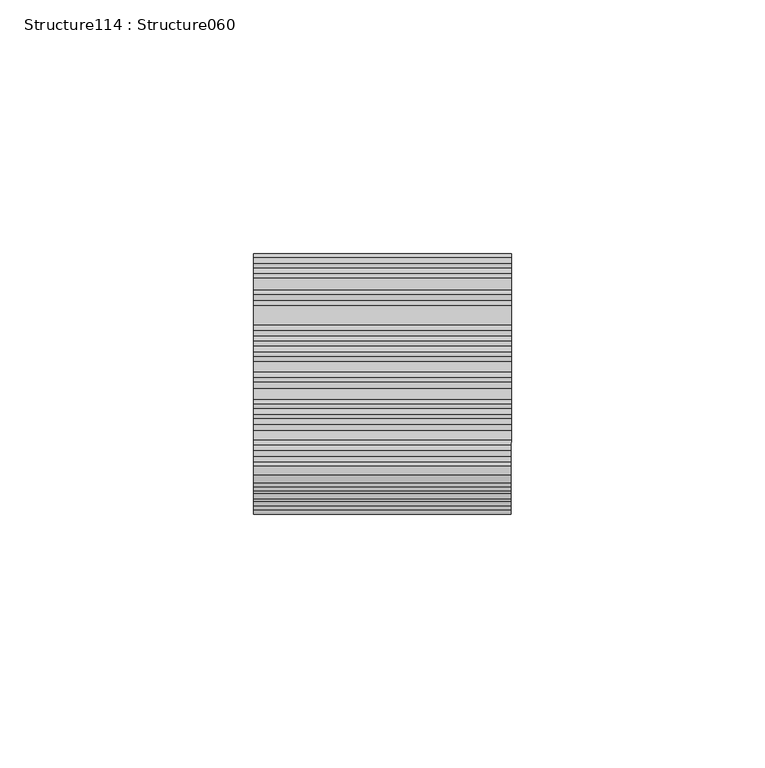
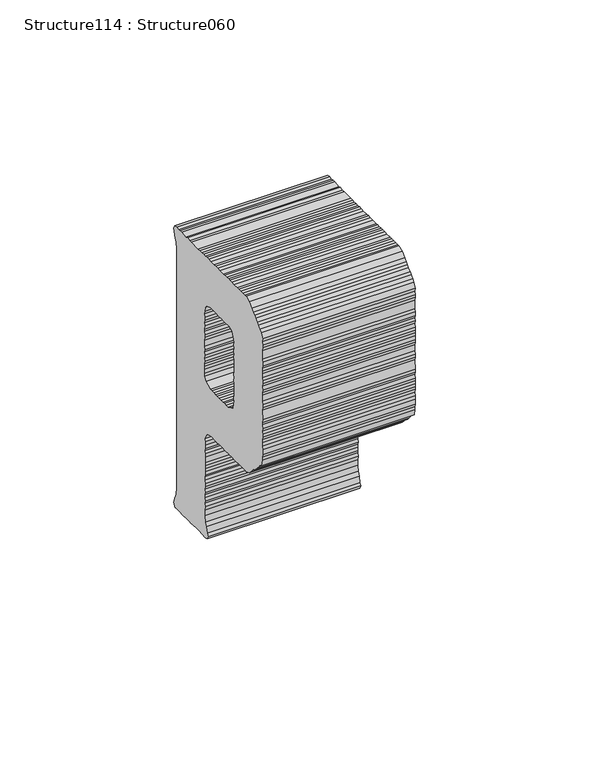
"""IFC4 building model written with IfcOpenShell, lengths in millimetres: proxy geometry, Structure114 : Structure060."""

from ifc_helpers import new_model, si_unit, frame, origin, place, context, project, spatial, polyline, outline, extrude, source, transform, mapped, element, save


def structure114_structure060_e718248d(model_context):
    return source(origin(), model_context, "Body", "SweptSolid", [
        extrude(outline(polyline([(1.9520053, 0.0), (3.1183694, 0.256899), (4.0274787, 0.1273821), (5.3272738, 0.0), (7.4077286, 0.0), (8.3171937, 0.256899), (9.226303, 0.0), (10.3976485, 0.256899), (11.1736827, 0.1273821), (12.3446724, 0.1273821), (13.516018, 0.0), (15.4630419, 0.1273821), (16.3725071, 0.1273821), (17.5434968, 0.256899), (18.7098608, 0.1273821), (19.7477754, 0.1273821), (20.5284353, 0.256899), (22.3470097, -0.5248282), (23.9086852, -1.9537844), (24.6847194, -2.8628937), (25.4703606, -3.5097668), (25.9894958, -4.1623329), (27.0270546, -4.9380113), (27.5461898, -5.7240084), (28.4552992, -6.6270688), (29.2363148, -7.2796349), (30.0119931, -8.9708273), (29.7550941, -10.1368356), (30.0119931, -11.3028439), (30.0119931, -12.0884851), (29.7550941, -13.2541376), (29.7550941, -16.2447692), (30.0119931, -17.2833954), (30.0119931, -18.5824788), (29.7550941, -19.4972812), (29.8835436, -20.4006974), (29.7550941, -21.4396795), (29.8835436, -22.7441001), (30.0119931, -23.6535653), (30.0119931, -24.6864985), (29.8835436, -25.7286829), (30.0119931, -27.0277663), (29.8835436, -28.0667483), (29.7550941, -28.9797716), (29.7550941, -31.0609381), (30.0119931, -32.0931596), (30.0119931, -33.264861), (29.7550941, -34.307757), (30.0119931, -37.425059), (29.8835436, -38.5932022), (29.7550941, -39.3731504), (30.0119931, -40.6722338), (29.8835436, -41.5777849), (30.0119931, -42.6199693), (30.0119931, -43.6585956), (29.8835436, -44.5680607), (29.7550941, -45.7376272), (29.8835436, -46.9096843), (30.0119931, -47.9479548), (30.0119931, -49.7665292), (29.7550941, -50.8090694), (29.7550941, -51.8455608), (29.3647643, -53.9228132), (28.3268497, -54.4458624), (27.8080702, -55.2218966), (26.2463948, -57.0401153), (25.5938287, -57.6926814), (24.5562699, -58.2121724), (23.2564748, -59.7681548), (22.3470097, -60.8103392), (20.5284353, -61.4589914), (19.7477754, -61.3298302), (18.5814114, -61.1963993), (16.3725071, -61.1963993), (15.3345925, -61.4589914), (14.2920522, -61.3298302), (13.2541376, -61.4589914), (12.473122, -61.3298302), (11.1736827, -61.3298302), (10.2642176, -61.1963993), (9.0978535, -61.4589914), (8.3171937, -61.3298302), (7.0173987, -61.1963993), (5.0703747, -61.1963993), (3.8990292, -61.4589914), (2.9899199, -61.3298302), (2.0804548, -61.3298302), (1.0425402, -61.1963993), (-0.2618804, -61.4589914), (-1.9470239, -61.9763475), (-2.4661592, -62.6289136), (-3.246819, -64.320106), (-2.9849385, -65.2292153), (-3.1183694, -66.5243847), (-2.9849385, -67.566925), (-3.246819, -68.4760343), (-2.9849385, -69.3854994), (-3.1183694, -70.6845828), (-3.1183694, -72.6362323), (-2.9849385, -73.6748586), (-3.1183694, -74.7134848), (-3.1183694, -75.7499762), (-2.9849385, -76.9216775), (-3.246819, -77.7016257), (-3.246819, -78.8694131), (-2.9849385, -79.9062602), (-3.1183694, -81.0818755), (-3.246819, -81.9870709), (-2.9849385, -83.1587722), (-3.246819, -83.9387204), (-3.246819, -84.9773466), (-3.1183694, -86.270737), (-3.246819, -87.0563782), (-2.9849385, -88.0950045), (-3.246819, -89.3940879), (-3.246819, -91.3421792), (-2.9849385, -93.4229899), (-2.3377097, -94.7163802), (-1.9470239, -96.7975467), (-1.4282446, -97.579274), (-1.9470239, -98.6157653), (-2.9849385, -98.8783574), (-5.1988244, -98.8783574), (-6.3651884, -98.7491962), (-7.2746536, -98.6157653), (-8.0553134, -98.6157653), (-10.3926672, -98.8783574), (-11.3021323, -98.8783574), (-12.3400469, -98.7491962), (-13.2491562, -98.8783574), (-14.2920522, -98.7491962), (-15.4584164, -98.8783574), (-16.5009566, -98.8783574), (-17.2769908, -98.7491962), (-19.4858951, -98.7491962), (-20.3953603, -98.8783574), (-21.1760201, -97.579274), (-20.9191211, -96.7975467), (-20.5287912, -95.7606995), (-20.009656, -94.4594812), (-19.8762251, -93.6798889), (-19.4858951, -91.3421792), (-19.4858951, -90.4327141), (-19.619326, -89.2667058), (-19.619326, -88.3519035), (-19.3574456, -87.3150563), (-19.619326, -86.1472689), (-19.619326, -85.2342456), (-19.3574456, -84.3286945), (-19.3574456, -83.2865101), (-19.4858951, -81.9870709), (-19.4858951, -81.0818755), (-19.3574456, -80.0393353), (-19.4858951, -79.130226), (-19.619326, -78.0876858), (-19.3574456, -76.7886024), (-19.619326, -75.8830513), (-19.619326, -74.970028), (-19.4858951, -73.9314017), (-19.4858951, -72.6362323), (-19.619326, -71.723209), (-19.4858951, -70.5572007), (-19.3574456, -69.5185745), (-19.4858951, -68.7386263), (-19.4858951, -67.7000001), (-19.3574456, -66.3952236), (-19.3574456, -64.4474881), (-19.4858951, -63.5380229), (-19.619326, -62.3684565), (-19.4858951, -61.1963993), (-19.3574456, -59.1212817), (-19.619326, -58.2121724), (-19.4858951, -57.0401153), (-19.619326, -56.136699), (-19.619326, -54.0558883), (-19.4858951, -53.1407302), (-19.4858951, -51.9747219), (-19.3574456, -50.9364514), (-19.619326, -49.8939112), (-19.3574456, -48.8570641), (-19.619326, -47.9479548), (-19.3574456, -46.6470923), (-19.619326, -45.6102451), (-19.4858951, -44.8285179), (-19.3574456, -43.5294345), (-19.3574456, -41.5777849), (-19.619326, -40.6722338), (-19.4858951, -39.3731504), (-19.3574456, -38.3302544), (-19.3574456, -37.2919839), (-19.4858951, -36.2551368), (-19.4858951, -32.2265905), (-19.3574456, -31.3135673), (-19.619326, -30.1457799), (-19.4858951, -29.2363148), (-19.619326, -27.9372314), (-19.3574456, -26.90074), (-19.4858951, -25.9916307), (-19.3574456, -25.0803865), (-19.3574456, -21.7001367), (-19.4858951, -20.6632895), (-19.4858951, -19.8812064), (-19.3574456, -18.71164), (-19.619326, -17.5438526), (-19.4858951, -16.6343875), (-19.4858951, -14.4258389), (-19.619326, -13.5170855), (-19.619326, -11.4362748), (-19.3574456, -10.5268097), (-19.619326, -9.2334193), (-19.3574456, -7.4091519), (-19.8762251, -5.0714422), (-20.266555, -4.032816), (-20.5287912, -2.9959688), (-20.9191211, -2.2142415), (-21.3044696, -1.0443193), (-20.5287912, 0.1273821), (-19.3574456, 0.256899), (-18.4479805, 0.0), (-17.4104217, 0.256899), (-16.5009566, 0.256899), (-14.1636027, 0.0), (-13.2491562, 0.256899), (-12.0827921, 0.0), (-11.0452333, 0.1273821), (-7.2746536, 0.0), (-6.1082895, 0.1273821), (-5.0653934, 0.0), (-4.0278346, 0.1273821), (-3.1183694, 0.0), (-1.9470239, 0.256899), (-1.0379146, 0.256899), (0.0, 0.0), (1.9520053, 0.0)]), holes=[polyline([(-2.5995901, -43.6585956), (0.0, -44.8285179), (0.9091093, -44.9580348), (2.0804548, -44.8285179), (3.1183694, -44.9580348), (3.8990292, -44.9580348), (5.0703747, -45.085061), (6.2367389, -44.9580348), (7.2742977, -45.085061), (8.0553133, -44.9580348), (9.0978535, -45.085061), (10.2642176, -44.9580348), (11.8258931, -44.1816448), (12.7353582, -43.7916707), (13.1207067, -41.9734521), (13.382587, -41.1917248), (13.1207067, -39.8926414), (13.382587, -38.8536594), (13.382587, -37.8168122), (13.2541376, -36.7728487), (13.382587, -35.7360015), (13.2541376, -34.8211992), (13.1207067, -33.784352), (13.382587, -32.7460816), (13.1207067, -31.5743802), (13.382587, -30.7979902), (13.2541376, -29.7558058), (13.2541376, -28.8463407), (13.382587, -27.8094935), (13.382587, -26.6377922), (13.1207067, -25.5995217), (13.382587, -24.4331576), (13.1207067, -23.6535653), (13.2541376, -22.4818639), (13.1207067, -21.3101626), (13.2541376, -20.4006974), (13.1207067, -19.3645619), (12.473122, -17.9356058), (12.0877735, -17.1538785), (10.3976485, -16.5016682), (8.3171937, -16.5016682), (7.0173987, -16.6343875), (6.1082894, -16.3739303), (4.9369438, -16.6343875), (4.1609097, -16.5016682), (3.1183694, -16.3739303), (-0.1284495, -16.3739303), (-2.0754734, -17.0264964), (-2.7280396, -17.8060888), (-3.1183694, -19.3645619), (-3.246819, -20.4006974), (-3.1183694, -21.4396795), (-3.1183694, -22.6152948), (-3.3752685, -23.6535653), (-3.1183694, -24.4331576), (-3.246819, -25.7286829), (-3.3752685, -26.6377922), (-3.1183694, -27.6806882), (-3.1183694, -28.5897975), (-3.246819, -29.6223749), (-3.246819, -31.7031855), (-3.1183694, -32.8791567), (-3.246819, -33.6555467), (-3.1183694, -34.8211992), (-3.246819, -35.9989494), (-3.1183694, -36.9023656), (-3.3752685, -38.0680181), (-3.246819, -38.8536594), (-3.3752685, -39.8926414), (-3.246819, -41.1917248), (-3.246819, -42.2299952), (-2.5995901, -43.6585956)])]), frame((-56111.4288051, 291465.0101438, -276.7221981), z_axis=(-0.9999998917542984, 0.00046528635450596156, 0.0), x_axis=(-0.00046528635450596156, -0.9999998917542984, 0.0)), (0.0, 0.0, 1.0), 50.8),
    ])


if __name__ == "__main__":
    model = new_model("IFC4")
    model_context = context("Model", 3, world=origin())
    ifc_project = project(units=[si_unit("LENGTHUNIT", "METRE", prefix="MILLI")], contexts=[model_context])
    site = spatial("IfcSite", under=ifc_project)
    building = spatial("IfcBuilding", under=site)
    placement = place(None, origin())
    structure114_structure060_shape = structure114_structure060_e718248d(model_context)
    element("IfcBuildingElementProxy", 1, Name="Structure114 : Structure060", ObjectType="Structure114 : Structure060", at=placement, inside=building, context=model_context, shape_type="MappedRepresentation", body=[
        mapped(structure114_structure060_shape, transform((0.0, 0.0, 0.0), x_axis=(1.0, 0.0, 0.0), y_axis=(0.0, 1.0, 0.0), z_axis=(0.0, 0.0, 1.0))),
    ])
    save(model, "model.ifc")

# Revit data of these elements
# Type "Structure114 : Structure060"
#   NameOverride = "Structure060"
# Element 1 (IfcBuildingElementProxy, "Structure114 : Structure060")
#   Materials on its faces: "BRUSHED ALUMINUM LETTERING"
# Materials
#   "BRUSHED ALUMINUM LETTERING": class "Unassigned", colour RGB 169 181 186, transparency 0, Cost = 0
